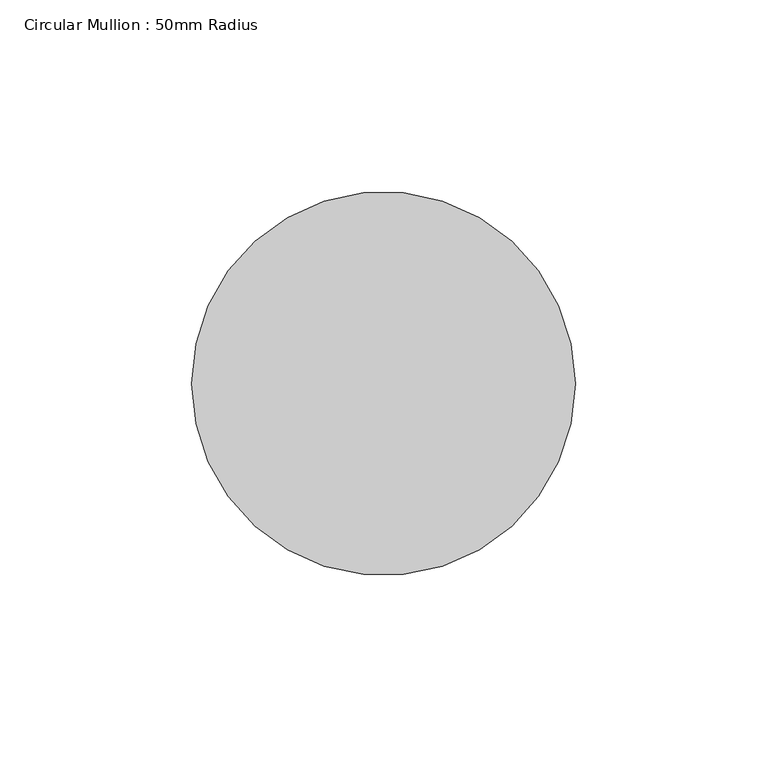
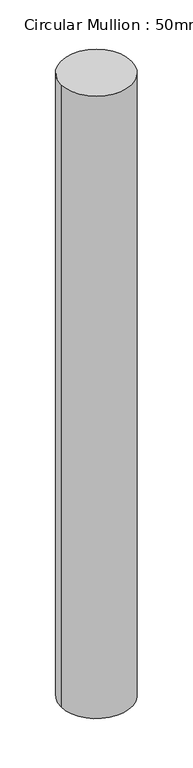
"""IFC4 building model written with IfcOpenShell, lengths in millimetres: member geometry, Circular Mullion : 50mm Radius."""

from ifc_helpers import new_model, si_unit, point, frame, origin, origin_2d, place, context, project, spatial, circle_curve, trimmed, segment, composite_curve, outline, extrude, source, transform, mapped, element, save


def circular_mullion_50mm_radius_05280f8c(model_context):
    return source(origin(), model_context, "Body", "SweptSolid", [
        extrude(outline(composite_curve([segment(trimmed(circle_curve(origin_2d(), 50.0), [point((50.0, 0.0))], [point((-50.0, 0.0))], False, "CARTESIAN"), True, "CONTINUOUS"), segment(trimmed(circle_curve(origin_2d(), 50.0), [point((-50.0, 0.0))], [point((50.0, 0.0))], False, "CARTESIAN"), True, "CONTINUOUS")], self_intersect=False)), frame((0.0, 0.0, -930.4302406), z_axis=(0.0, 0.0, 1.0), x_axis=(1.0, 0.0, 0.0)), (0.0, 0.0, 1.0), 930.4302406),
    ])


if __name__ == "__main__":
    model = new_model("IFC4")
    model_context = context("Model", 3, world=origin())
    ifc_project = project(units=[si_unit("LENGTHUNIT", "METRE", prefix="MILLI")], contexts=[model_context])
    site = spatial("IfcSite", under=ifc_project)
    building = spatial("IfcBuilding", under=site)
    placement = place(None, origin())
    circular_mullion_50mm_radius_shape = circular_mullion_50mm_radius_05280f8c(model_context)
    element("IfcMember", 1, ObjectType="Circular Mullion : 50mm Radius", at=placement, inside=building, context=model_context, shape_type="MappedRepresentation", body=[
        mapped(circular_mullion_50mm_radius_shape, transform((0.0, 0.0, 0.0), x_axis=(1.0, 0.0, 0.0), y_axis=(0.0, 1.0, 0.0), z_axis=(0.0, 0.0, 1.0))),
    ])
    save(model, "model.ifc")

# Revit data of these elements
# Type "Circular Mullion : 50mm Radius"
#   built-in parameter 1007350 = 0.164042 (stored number, unit not read)
# Element 1 (IfcMember, "Circular Mullion : 50mm Radius")
#   Materials on its faces: "Aluminium"
# Materials
#   "Aluminium": class "Metal", colour RGB 247 247 247, transparency 0, Description = "Aluminium 6061", Cost = 0
